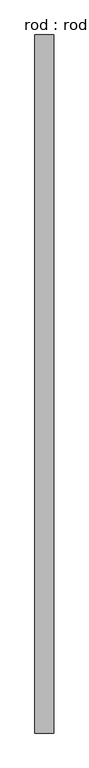
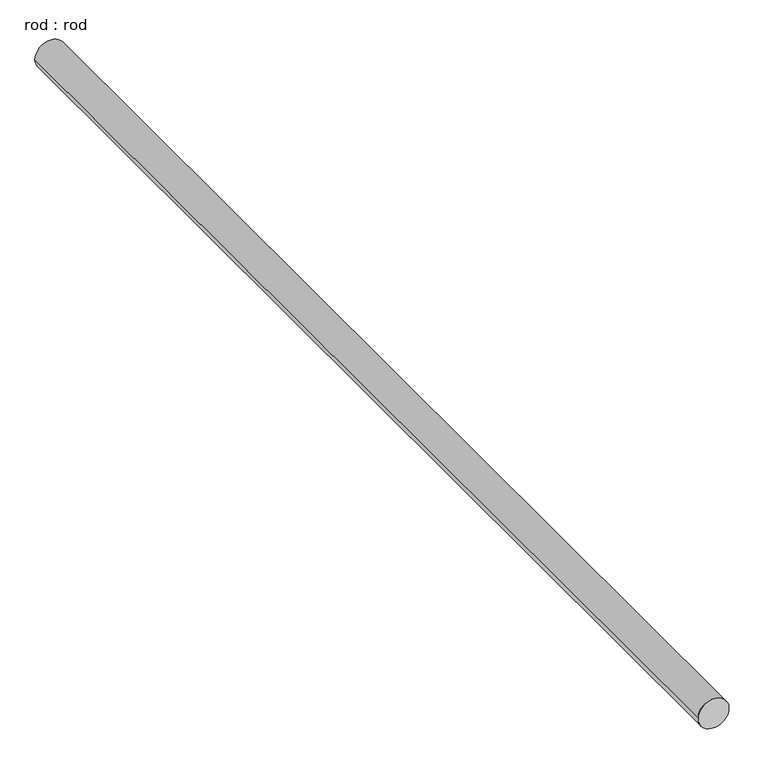
"""IFC4 building model written with IfcOpenShell, lengths in millimetres: proxy geometry, rod : rod."""

from ifc_helpers import new_model, si_unit, point, frame, frame_2d, origin, place, context, project, spatial, circle_curve, trimmed, segment, composite_curve, outline, extrude, source, transform, mapped, element, save


def rod_rod_03e20f27(model_context):
    return source(origin(), model_context, "Body", "SweptSolid", [
        extrude(outline(composite_curve([segment(trimmed(circle_curve(frame_2d((0.0108462, 0.0)), 200.0), [point((0.0108462, 200.0))], [point((0.0108462, -200.0))], False, "CARTESIAN"), True, "CONTINUOUS"), segment(trimmed(circle_curve(frame_2d((0.0108462, 0.0)), 200.0), [point((0.0108462, -200.0))], [point((0.0108462, 200.0))], False, "CARTESIAN"), True, "CONTINUOUS")], self_intersect=False)), frame((0.0, -3351.7158291, 0.0), z_axis=(0.0, 1.0, 0.0), x_axis=(0.0, 0.0, 1.0)), (0.0, 0.0, 1.0), 14888.8888889),
    ])


if __name__ == "__main__":
    model = new_model("IFC4")
    model_context = context("Model", 3, world=origin())
    ifc_project = project(units=[si_unit("LENGTHUNIT", "METRE", prefix="MILLI")], contexts=[model_context])
    site = spatial("IfcSite", under=ifc_project)
    building = spatial("IfcBuilding", under=site)
    placement = place(None, origin())
    rod_rod_shape = rod_rod_03e20f27(model_context)
    element("IfcBuildingElementProxy", 1, Name="rod : rod", ObjectType="rod : rod", at=placement, inside=building, context=model_context, shape_type="MappedRepresentation", body=[
        mapped(rod_rod_shape, transform((0.0, 0.0, 0.0), x_axis=(1.0, 0.0, 0.0), y_axis=(0.0, 1.0, 0.0), z_axis=(0.0, 0.0, 1.0))),
    ])
    save(model, "model.ifc")

# Revit data of these elements
# Type "rod : rod"
#   Default Elevation = 0
